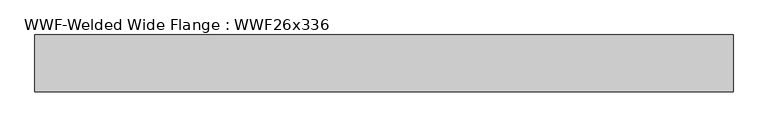
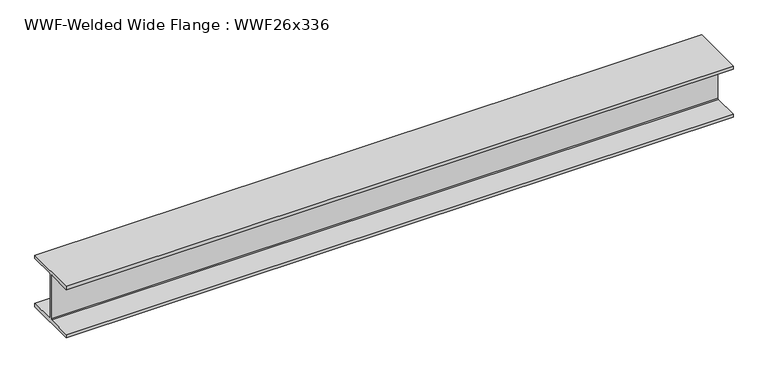
"""IFC4 building model written with IfcOpenShell, lengths in millimetres: beam geometry, WWF-Welded Wide Flange : WWF26x336."""

from ifc_helpers import new_model, si_unit, frame, origin, place, context, project, spatial, polyline, outline, extrude, source, transform, mapped, element, save


def wwf_welded_wide_flange_wwf26x336_18b7577a(model_context):
    return source(origin(), model_context, "Body", "SweptSolid", [
        extrude(outline(polyline([(324.993, -284.988), (324.993, -324.993), (-324.993, -324.993), (-324.993, -284.988), (-20.6375, -284.988), (-9.9949, -274.3454), (-9.9949, 274.3454), (-20.6375, 284.988), (-324.993, 284.988), (-324.993, 324.993), (324.993, 324.993), (324.993, 284.988), (20.6375, 284.988), (9.9949, 274.3454), (9.9949, -274.3454), (20.6375, -284.988), (324.993, -284.988)])), frame((-3827.7582557, 0.0, 0.0), z_axis=(1.0, 0.0, 0.0), x_axis=(0.0, 1.0, 0.0)), (0.0, 0.0, 1.0), 7985.2412398),
    ])


if __name__ == "__main__":
    model = new_model("IFC4")
    model_context = context("Model", 3, world=origin())
    ifc_project = project(units=[si_unit("LENGTHUNIT", "METRE", prefix="MILLI")], contexts=[model_context])
    site = spatial("IfcSite", under=ifc_project)
    building = spatial("IfcBuilding", under=site)
    placement = place(None, origin())
    wwf_welded_wide_flange_wwf26x336_shape = wwf_welded_wide_flange_wwf26x336_18b7577a(model_context)
    element("IfcBeam", 1, ObjectType="WWF-Welded Wide Flange : WWF26x336", at=placement, inside=building, context=model_context, shape_type="MappedRepresentation", body=[
        mapped(wwf_welded_wide_flange_wwf26x336_shape, transform((0.0, 0.0, 0.0), x_axis=(1.0, 0.0, 0.0), y_axis=(0.0, 1.0, 0.0), z_axis=(0.0, 0.0, 1.0))),
    ])
    save(model, "model.ifc")

# Revit data of these elements
# Type "WWF-Welded Wide Flange : WWF26x336"
#   Assembly Code = "B10"
#   Nominal d = "12"
#   W = 336
#   Length [instance default] = 1524 mm
#   bf = 649.986 mm
#   d = 649.986 mm
#   k = 20.638 mm
#   tf = 40.005 mm
#   tw = 19.99 mm
#   A = 0.0635483 m²
#   Structural Material [instance default] = Steel ASTM A572
# Element 1 (IfcBeam, "WWF-Welded Wide Flange : WWF26x336")
#   Structural Material = Metal - Steel 43-275
#   Materials on its faces: "Metal - Steel 43-275"
# Materials
#   "Steel ASTM A572": class "Metal", colour RGB 247 247 247, transparency 0, Description = "Structural steel, high strength low alloy, ASTM - A572 - 50", Cost = 0
#   "Metal - Steel 43-275": class "Metal", colour RGB 247 247 247, transparency 0, Cost = 0
